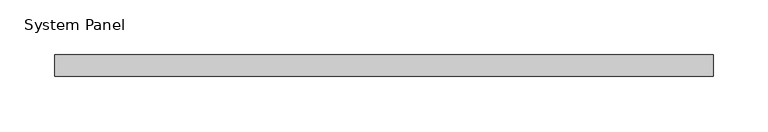
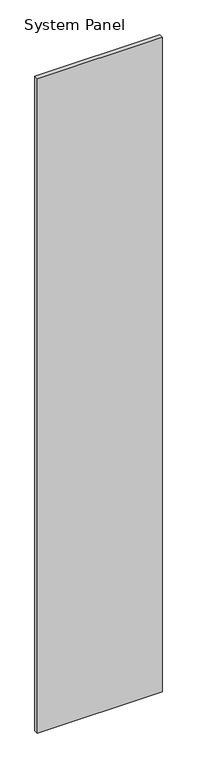
"""IFC4 building model written with IfcOpenShell, lengths in millimetres: plate geometry, System Panel : WWm-Glass-20mm-10mmOffset."""

import ifcopenshell
import ifcopenshell.guid

model = None  # the IFC model being written
_history = None  # IfcOwnerHistory: only IFC2X3 demands one
_inside = {}  # id of a spatial element -> (the spatial element, [elements in it])
_under = {}  # id of a project, library or spatial element -> (it, [spatial elements below it])
_declared = {}  # id of a project -> (the project, [libraries it declares])
_typed = {}  # id of a type object -> (the type object, [elements of that type])
_made_of = {}  # id of a material, layer set ... -> (it, [elements and type objects made of it])


def new_model(schema):
    """Start an empty IFC model of exactly this schema.

    Asked for "IFC4X3", IfcOpenShell would pick the latest addendum, in which some entities
    have other attributes; the version numbers below select the first issue.
    IFC2X3 requires an IfcOwnerHistory on every rooted entity: one is made here for all.
    """
    global model, _history
    if schema == "IFC4X3":
        model = ifcopenshell.file(schema_version=(4, 3, 0, 0))
    else:
        model = ifcopenshell.file(schema=schema)
    _inside.clear()
    _under.clear()
    _declared.clear()
    _typed.clear()
    _made_of.clear()
    _history = None
    if model.schema == "IFC2X3":
        org = make("IfcOrganization", Name="unknown")
        user = make(
            "IfcPersonAndOrganization",
            ThePerson=make("IfcPerson", FamilyName="unknown"),
            TheOrganization=org,
        )
        app = make(
            "IfcApplication",
            ApplicationDeveloper=org,
            Version="unknown",
            ApplicationFullName="unknown",
            ApplicationIdentifier="unknown",
        )
        _history = make(
            "IfcOwnerHistory",
            OwningUser=user,
            OwningApplication=app,
            ChangeAction="ADDED",
            CreationDate=0,
        )
    return model


def make(cls, **values):
    """One entity of the class cls with the attributes given. An attribute that is None is left unset."""
    return model.create_entity(
        cls, **{name: value for name, value in values.items() if value is not None}
    )


def rooted(cls, **values):
    """An entity with a GlobalId (a new one), such as an element, a storey or a relation."""
    return make(cls, GlobalId=ifcopenshell.guid.new(), OwnerHistory=_history, **values)


def si_unit(unit_type, name, prefix=None):
    """IfcSIUnit, for example si_unit("LENGTHUNIT", "METRE", prefix="MILLI")."""
    return make("IfcSIUnit", UnitType=unit_type, Prefix=prefix, Name=name)


def assignment(units):
    """IfcUnitAssignment: the units of a project."""
    return None if units is None else make("IfcUnitAssignment", Units=units)


def point(xyz):
    """IfcCartesianPoint."""
    return None if xyz is None else make("IfcCartesianPoint", Coordinates=xyz)


def direction(xyz):
    """IfcDirection."""
    return None if xyz is None else make("IfcDirection", DirectionRatios=xyz)


def frame(location, z_axis=None, x_axis=None):
    """IfcAxis2Placement3D, a coordinate frame: its origin and axes. An axis left out is left unset."""
    return make(
        "IfcAxis2Placement3D",
        Location=point(location),
        Axis=direction(z_axis),
        RefDirection=direction(x_axis),
    )


def origin():
    """The frame at (0, 0, 0) with its axes left unset."""
    return frame((0.0, 0.0, 0.0))


def origin_with_axes():
    """The frame at (0, 0, 0) with the z axis (0, 0, 1) and the x axis (1, 0, 0) written out."""
    return frame((0.0, 0.0, 0.0), z_axis=(0.0, 0.0, 1.0), x_axis=(1.0, 0.0, 0.0))


def place(relative_to, where):
    """IfcLocalPlacement: puts the frame where relative to a parent placement (None: the world)."""
    return make(
        "IfcLocalPlacement", PlacementRelTo=relative_to, RelativePlacement=where
    )


def context(
    kind, dimensions, precision=None, world=None, true_north=None, identifier=None
):
    """IfcGeometricRepresentationContext, for example the 3D "Model" context."""
    return make(
        "IfcGeometricRepresentationContext",
        ContextIdentifier=identifier,
        ContextType=kind,
        CoordinateSpaceDimension=dimensions,
        Precision=precision,
        WorldCoordinateSystem=world,
        TrueNorth=true_north,
    )


def project(units=None, contexts=None):
    """IfcProject with its units and contexts."""
    return rooted(
        "IfcProject",
        Name="project",
        RepresentationContexts=contexts,
        UnitsInContext=assignment(units),
    )


def spatial(cls, under=None, at=None, **own):
    """A site, building, storey or space (cls), placed at a placement, below another one or the project."""
    s = rooted(cls, ObjectPlacement=at, **own)
    if under is not None:
        _under.setdefault(under.id(), (under, []))[1].append(s)
    return s


def polyline(points):
    """IfcPolyline through the points."""
    return make("IfcPolyline", Points=[point(p) for p in points])


def outline(outer, holes=None, kind="AREA"):
    """IfcArbitraryClosedProfileDef: a profile drawn as a closed curve; with holes, ...WithVoids."""
    if holes is None:
        return make("IfcArbitraryClosedProfileDef", ProfileType=kind, OuterCurve=outer)
    return make(
        "IfcArbitraryProfileDefWithVoids",
        ProfileType=kind,
        OuterCurve=outer,
        InnerCurves=holes,
    )


def extrude(swept, where, along, depth):
    """IfcExtrudedAreaSolid: the profile swept, set in the frame where, extruded along a direction by depth."""
    return make(
        "IfcExtrudedAreaSolid",
        SweptArea=swept,
        Position=where,
        ExtrudedDirection=direction(along),
        Depth=depth,
    )


def shape(context_of_items, identifier, shape_type, items):
    """IfcShapeRepresentation: the items that make up one representation, for example the "Body"."""
    return make(
        "IfcShapeRepresentation",
        ContextOfItems=context_of_items,
        RepresentationIdentifier=identifier,
        RepresentationType=shape_type,
        Items=items,
    )


def source(mapping_origin, context_of_items, identifier, shape_type, items):
    """IfcRepresentationMap: a shape defined once, which mapped items show again and again."""
    return make(
        "IfcRepresentationMap",
        MappingOrigin=mapping_origin,
        MappedRepresentation=shape(context_of_items, identifier, shape_type, items),
    )


def transform(
    local_origin,
    x_axis=None,
    y_axis=None,
    z_axis=None,
    scale=None,
    scale2=None,
    scale3=None,
    uniform=True,
):
    """IfcCartesianTransformationOperator3D, or its non-uniform kind. x_axis, y_axis, z_axis: its Axis1, 2, 3."""
    if uniform:
        return make(
            "IfcCartesianTransformationOperator3D",
            Axis1=direction(x_axis),
            Axis2=direction(y_axis),
            LocalOrigin=point(local_origin),
            Scale=scale,
            Axis3=direction(z_axis),
        )
    return make(
        "IfcCartesianTransformationOperator3DnonUniform",
        Axis1=direction(x_axis),
        Axis2=direction(y_axis),
        LocalOrigin=point(local_origin),
        Scale=scale,
        Axis3=direction(z_axis),
        Scale2=scale2,
        Scale3=scale3,
    )


def mapped(mapping_source, mapping_target):
    """IfcMappedItem: shows the shape of a source again, moved by a transform."""
    return make(
        "IfcMappedItem", MappingSource=mapping_source, MappingTarget=mapping_target
    )


def made_of(thing, what):
    """Note that an element or type object is made of a material, layer set ...; save() writes the relation."""
    if what is not None:
        _made_of.setdefault(what.id(), (what, []))[1].append(thing)
    return thing


def element(
    cls,
    number,
    at=None,
    inside=None,
    cuts=None,
    type_object=None,
    material=None,
    context=None,
    identifier="Body",
    shape_type=None,
    held_by="IfcProductDefinitionShape",
    body=None,
    shapes=None,
    **own,
):
    """One element of the class cls, such as IfcWall. Its Tag is "e" and its number.

    at: its placement. inside: the storey or other place that contains it. cuts: it is an
    opening in that element (IfcRelVoidsElement). A single representation is given by context,
    identifier, shape_type and body (its items); several are given by shapes. held_by: the class
    of the entity that holds the representations. save() writes the other relations.
    """
    e = rooted(cls, Tag="e%d" % number, ObjectPlacement=at, **own)
    if body is not None:
        shapes = [shape(context, identifier, shape_type, body)]
    if shapes is not None:
        e.Representation = make(held_by, Representations=shapes)
    if inside is not None:
        _inside.setdefault(inside.id(), (inside, []))[1].append(e)
    if cuts is not None:
        rooted(
            "IfcRelVoidsElement", RelatingBuildingElement=cuts, RelatedOpeningElement=e
        )
    if type_object is not None:
        _typed.setdefault(type_object.id(), (type_object, []))[1].append(e)
    return made_of(e, material)


def aggregate(whole, parts):
    """IfcRelAggregates: a whole, such as a stair, and the parts it consists of."""
    return rooted("IfcRelAggregates", RelatingObject=whole, RelatedObjects=parts)


def save(model, path):
    """Write the relations noted so far, then the file.

    IfcRelAggregates (storeys below a building ...), IfcRelContainedInSpatialStructure (elements
    in a storey), IfcRelDefinesByType, IfcRelAssociatesMaterial and IfcRelDeclares: one each for
    every whole, place, type object, material and project.
    """
    for whole, parts in _under.values():
        aggregate(whole, parts)
    for where, things in _inside.values():
        rooted(
            "IfcRelContainedInSpatialStructure",
            RelatedElements=things,
            RelatingStructure=where,
        )
    for kind, things in _typed.values():
        rooted("IfcRelDefinesByType", RelatedObjects=things, RelatingType=kind)
    for what, things in _made_of.values():
        rooted("IfcRelAssociatesMaterial", RelatedObjects=things, RelatingMaterial=what)
    for by, libraries in _declared.values():
        rooted("IfcRelDeclares", RelatingContext=by, RelatedDefinitions=libraries)
    model.write(path)


def system_panel_bca5d789(model_context):
    return source(origin(), model_context, "Body", "SweptSolid", [
        extrude(outline(polyline([(302.0, 0.0), (-302.0, 0.0), (-302.0, 20.0), (302.0, 20.0), (302.0, 0.0)])), origin_with_axes(), (0.0, 0.0, 1.0), 3350.0),
    ])


if __name__ == "__main__":
    model = new_model("IFC4")
    model_context = context("Model", 3, world=origin())
    ifc_project = project(units=[si_unit("LENGTHUNIT", "METRE", prefix="MILLI")], contexts=[model_context])
    site = spatial("IfcSite", under=ifc_project)
    building = spatial("IfcBuilding", under=site)
    placement = place(None, origin())
    system_panel_shape = system_panel_bca5d789(model_context)
    element("IfcPlate", 1, ObjectType="System Panel : WWm-Glass-20mm-10mmOffset", at=placement, inside=building, context=model_context, shape_type="MappedRepresentation", body=[
        mapped(system_panel_shape, transform((0.0, 0.0, 0.0), x_axis=(1.0, 0.0, 0.0), y_axis=(0.0, 1.0, 0.0), z_axis=(0.0, 0.0, 1.0))),
    ])
    save(model, "model.ifc")

# Revit data of these elements
# Type "System Panel : WWm-Glass-20mm-10mmOffset"
#   Finish = ""
# Element 1 (IfcPlate, "System Panel : WWm-Glass-20mm-10mmOffset")
#   Materials on its faces: "WW-EC-GL-Storefront"
# Materials
#   "WW-EC-GL-Storefront": class "Glass", colour RGB 236 240 239, transparency 0.85, Description = "Storefront Glass", Cost = 0
